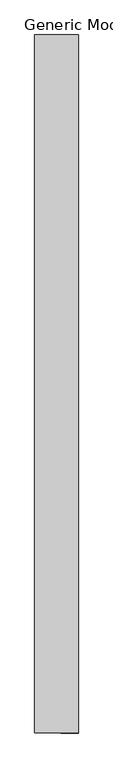
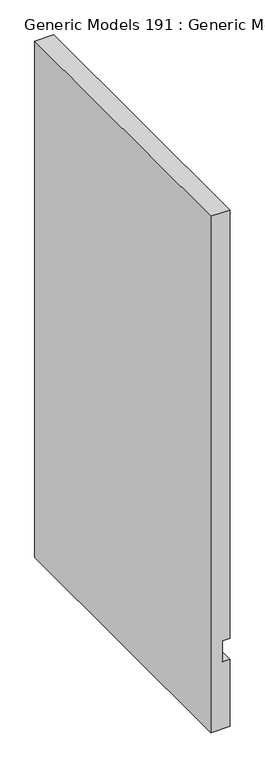
"""IFC4 building model written with IfcOpenShell, lengths in millimetres: proxy geometry, Generic Models 191 : Generic Models 1."""

import ifcopenshell
import ifcopenshell.guid

model = None  # the IFC model being written
_history = None  # IfcOwnerHistory: only IFC2X3 demands one
_inside = {}  # id of a spatial element -> (the spatial element, [elements in it])
_under = {}  # id of a project, library or spatial element -> (it, [spatial elements below it])
_declared = {}  # id of a project -> (the project, [libraries it declares])
_typed = {}  # id of a type object -> (the type object, [elements of that type])
_made_of = {}  # id of a material, layer set ... -> (it, [elements and type objects made of it])


def new_model(schema):
    """Start an empty IFC model of exactly this schema.

    Asked for "IFC4X3", IfcOpenShell would pick the latest addendum, in which some entities
    have other attributes; the version numbers below select the first issue.
    IFC2X3 requires an IfcOwnerHistory on every rooted entity: one is made here for all.
    """
    global model, _history
    if schema == "IFC4X3":
        model = ifcopenshell.file(schema_version=(4, 3, 0, 0))
    else:
        model = ifcopenshell.file(schema=schema)
    _inside.clear()
    _under.clear()
    _declared.clear()
    _typed.clear()
    _made_of.clear()
    _history = None
    if model.schema == "IFC2X3":
        org = make("IfcOrganization", Name="unknown")
        user = make(
            "IfcPersonAndOrganization",
            ThePerson=make("IfcPerson", FamilyName="unknown"),
            TheOrganization=org,
        )
        app = make(
            "IfcApplication",
            ApplicationDeveloper=org,
            Version="unknown",
            ApplicationFullName="unknown",
            ApplicationIdentifier="unknown",
        )
        _history = make(
            "IfcOwnerHistory",
            OwningUser=user,
            OwningApplication=app,
            ChangeAction="ADDED",
            CreationDate=0,
        )
    return model


def make(cls, **values):
    """One entity of the class cls with the attributes given. An attribute that is None is left unset."""
    return model.create_entity(
        cls, **{name: value for name, value in values.items() if value is not None}
    )


def rooted(cls, **values):
    """An entity with a GlobalId (a new one), such as an element, a storey or a relation."""
    return make(cls, GlobalId=ifcopenshell.guid.new(), OwnerHistory=_history, **values)


def si_unit(unit_type, name, prefix=None):
    """IfcSIUnit, for example si_unit("LENGTHUNIT", "METRE", prefix="MILLI")."""
    return make("IfcSIUnit", UnitType=unit_type, Prefix=prefix, Name=name)


def assignment(units):
    """IfcUnitAssignment: the units of a project."""
    return None if units is None else make("IfcUnitAssignment", Units=units)


def point(xyz):
    """IfcCartesianPoint."""
    return None if xyz is None else make("IfcCartesianPoint", Coordinates=xyz)


def direction(xyz):
    """IfcDirection."""
    return None if xyz is None else make("IfcDirection", DirectionRatios=xyz)


def frame(location, z_axis=None, x_axis=None):
    """IfcAxis2Placement3D, a coordinate frame: its origin and axes. An axis left out is left unset."""
    return make(
        "IfcAxis2Placement3D",
        Location=point(location),
        Axis=direction(z_axis),
        RefDirection=direction(x_axis),
    )


def origin():
    """The frame at (0, 0, 0) with its axes left unset."""
    return frame((0.0, 0.0, 0.0))


def place(relative_to, where):
    """IfcLocalPlacement: puts the frame where relative to a parent placement (None: the world)."""
    return make(
        "IfcLocalPlacement", PlacementRelTo=relative_to, RelativePlacement=where
    )


def context(
    kind, dimensions, precision=None, world=None, true_north=None, identifier=None
):
    """IfcGeometricRepresentationContext, for example the 3D "Model" context."""
    return make(
        "IfcGeometricRepresentationContext",
        ContextIdentifier=identifier,
        ContextType=kind,
        CoordinateSpaceDimension=dimensions,
        Precision=precision,
        WorldCoordinateSystem=world,
        TrueNorth=true_north,
    )


def project(units=None, contexts=None):
    """IfcProject with its units and contexts."""
    return rooted(
        "IfcProject",
        Name="project",
        RepresentationContexts=contexts,
        UnitsInContext=assignment(units),
    )


def spatial(cls, under=None, at=None, **own):
    """A site, building, storey or space (cls), placed at a placement, below another one or the project."""
    s = rooted(cls, ObjectPlacement=at, **own)
    if under is not None:
        _under.setdefault(under.id(), (under, []))[1].append(s)
    return s


def polyline(points):
    """IfcPolyline through the points."""
    return make("IfcPolyline", Points=[point(p) for p in points])


def outline(outer, holes=None, kind="AREA"):
    """IfcArbitraryClosedProfileDef: a profile drawn as a closed curve; with holes, ...WithVoids."""
    if holes is None:
        return make("IfcArbitraryClosedProfileDef", ProfileType=kind, OuterCurve=outer)
    return make(
        "IfcArbitraryProfileDefWithVoids",
        ProfileType=kind,
        OuterCurve=outer,
        InnerCurves=holes,
    )


def extrude(swept, where, along, depth):
    """IfcExtrudedAreaSolid: the profile swept, set in the frame where, extruded along a direction by depth."""
    return make(
        "IfcExtrudedAreaSolid",
        SweptArea=swept,
        Position=where,
        ExtrudedDirection=direction(along),
        Depth=depth,
    )


def shape(context_of_items, identifier, shape_type, items):
    """IfcShapeRepresentation: the items that make up one representation, for example the "Body"."""
    return make(
        "IfcShapeRepresentation",
        ContextOfItems=context_of_items,
        RepresentationIdentifier=identifier,
        RepresentationType=shape_type,
        Items=items,
    )


def source(mapping_origin, context_of_items, identifier, shape_type, items):
    """IfcRepresentationMap: a shape defined once, which mapped items show again and again."""
    return make(
        "IfcRepresentationMap",
        MappingOrigin=mapping_origin,
        MappedRepresentation=shape(context_of_items, identifier, shape_type, items),
    )


def transform(
    local_origin,
    x_axis=None,
    y_axis=None,
    z_axis=None,
    scale=None,
    scale2=None,
    scale3=None,
    uniform=True,
):
    """IfcCartesianTransformationOperator3D, or its non-uniform kind. x_axis, y_axis, z_axis: its Axis1, 2, 3."""
    if uniform:
        return make(
            "IfcCartesianTransformationOperator3D",
            Axis1=direction(x_axis),
            Axis2=direction(y_axis),
            LocalOrigin=point(local_origin),
            Scale=scale,
            Axis3=direction(z_axis),
        )
    return make(
        "IfcCartesianTransformationOperator3DnonUniform",
        Axis1=direction(x_axis),
        Axis2=direction(y_axis),
        LocalOrigin=point(local_origin),
        Scale=scale,
        Axis3=direction(z_axis),
        Scale2=scale2,
        Scale3=scale3,
    )


def mapped(mapping_source, mapping_target):
    """IfcMappedItem: shows the shape of a source again, moved by a transform."""
    return make(
        "IfcMappedItem", MappingSource=mapping_source, MappingTarget=mapping_target
    )


def made_of(thing, what):
    """Note that an element or type object is made of a material, layer set ...; save() writes the relation."""
    if what is not None:
        _made_of.setdefault(what.id(), (what, []))[1].append(thing)
    return thing


def element(
    cls,
    number,
    at=None,
    inside=None,
    cuts=None,
    type_object=None,
    material=None,
    context=None,
    identifier="Body",
    shape_type=None,
    held_by="IfcProductDefinitionShape",
    body=None,
    shapes=None,
    **own,
):
    """One element of the class cls, such as IfcWall. Its Tag is "e" and its number.

    at: its placement. inside: the storey or other place that contains it. cuts: it is an
    opening in that element (IfcRelVoidsElement). A single representation is given by context,
    identifier, shape_type and body (its items); several are given by shapes. held_by: the class
    of the entity that holds the representations. save() writes the other relations.
    """
    e = rooted(cls, Tag="e%d" % number, ObjectPlacement=at, **own)
    if body is not None:
        shapes = [shape(context, identifier, shape_type, body)]
    if shapes is not None:
        e.Representation = make(held_by, Representations=shapes)
    if inside is not None:
        _inside.setdefault(inside.id(), (inside, []))[1].append(e)
    if cuts is not None:
        rooted(
            "IfcRelVoidsElement", RelatingBuildingElement=cuts, RelatedOpeningElement=e
        )
    if type_object is not None:
        _typed.setdefault(type_object.id(), (type_object, []))[1].append(e)
    return made_of(e, material)


def aggregate(whole, parts):
    """IfcRelAggregates: a whole, such as a stair, and the parts it consists of."""
    return rooted("IfcRelAggregates", RelatingObject=whole, RelatedObjects=parts)


def save(model, path):
    """Write the relations noted so far, then the file.

    IfcRelAggregates (storeys below a building ...), IfcRelContainedInSpatialStructure (elements
    in a storey), IfcRelDefinesByType, IfcRelAssociatesMaterial and IfcRelDeclares: one each for
    every whole, place, type object, material and project.
    """
    for whole, parts in _under.values():
        aggregate(whole, parts)
    for where, things in _inside.values():
        rooted(
            "IfcRelContainedInSpatialStructure",
            RelatedElements=things,
            RelatingStructure=where,
        )
    for kind, things in _typed.values():
        rooted("IfcRelDefinesByType", RelatedObjects=things, RelatingType=kind)
    for what, things in _made_of.values():
        rooted("IfcRelAssociatesMaterial", RelatedObjects=things, RelatingMaterial=what)
    for by, libraries in _declared.values():
        rooted("IfcRelDeclares", RelatingContext=by, RelatedDefinitions=libraries)
    model.write(path)


def generic_models_191_generic_models_1_83decbcf(model_context):
    return source(origin(), model_context, "Body", "SweptSolid", [
        extrude(outline(polyline([(7.9375, 47261.4625), (7.9375, 47337.6625), (291.1195631, 47337.6625), (291.1195631, 47307.5), (380.0195631, 47307.5), (380.0195631, 47337.6625), (2188.2204978, 47337.6625), (2188.2204978, 47261.4625), (7.9375, 47261.4625)])), frame((0.0, 0.0, 0.0), z_axis=(0.0, 1.0, 0.0), x_axis=(0.0, 0.0, 1.0)), (0.0, 0.0, 1.0), 1219.2),
    ])


if __name__ == "__main__":
    model = new_model("IFC4")
    model_context = context("Model", 3, world=origin())
    ifc_project = project(units=[si_unit("LENGTHUNIT", "METRE", prefix="MILLI")], contexts=[model_context])
    site = spatial("IfcSite", under=ifc_project)
    building = spatial("IfcBuilding", under=site)
    placement = place(None, origin())
    generic_models_191_generic_models_1_shape = generic_models_191_generic_models_1_83decbcf(model_context)
    element("IfcBuildingElementProxy", 1, Name="Generic Models 191 : Generic Models 1", ObjectType="Generic Models 191 : Generic Models 1", at=placement, inside=building, context=model_context, shape_type="MappedRepresentation", body=[
        mapped(generic_models_191_generic_models_1_shape, transform((0.0, 0.0, 0.0), x_axis=(1.0, 0.0, 0.0), y_axis=(0.0, 1.0, 0.0), z_axis=(0.0, 0.0, 1.0))),
    ])
    save(model, "model.ifc")

# Revit data of these elements
# Element 1 (IfcBuildingElementProxy, "Generic Models 191 : Generic Models 1")
#   Materials on its faces: "(S) SOUND BATT. INSULATION (THICKNESS TO MATCH WALL DEPTH)"
# Materials
#   "(S) SOUND BATT. INSULATION (THICKNESS TO MATCH WALL DEPTH)": class "Unassigned", colour RGB 255 255 255, transparency 0, Cost = 0
